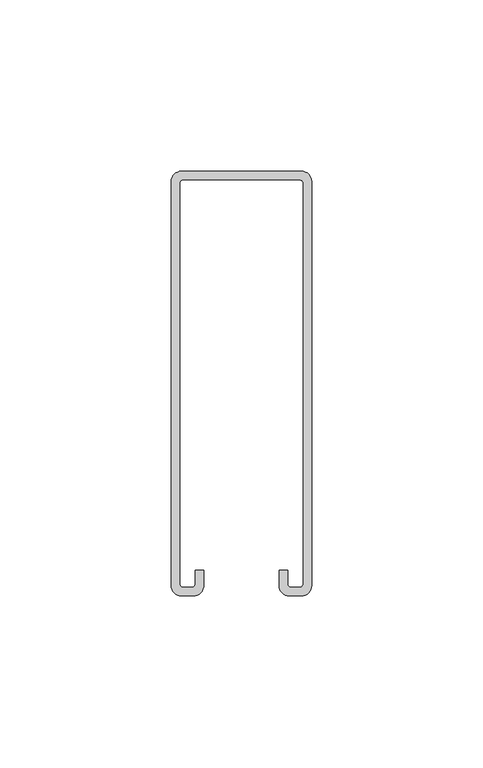
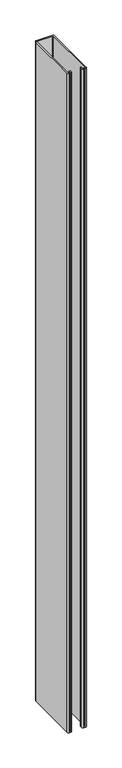
"""IFC4 building model written with IfcOpenShell, lengths in millimetres: proxy geometry, TN_Профиль монтажный : Профиль монтажный 41x124x2,5-6000."""

from ifc_helpers import new_model, si_unit, point, frame_2d, origin, origin_with_axes, place, context, project, spatial, polyline, circle_curve, trimmed, segment, composite_curve, outline, extrude, source, transform, mapped, element, save


def generic_models_93cc7051(model_context):
    return source(origin(), model_context, "Body", "SweptSolid", [
        extrude(outline(composite_curve([segment(trimmed(circle_curve(frame_2d((-17.5, -3.0)), 3.0), [point((-20.5, -3.0))], [point((-17.5, 0.0))], False, "CARTESIAN"), True, "CONTINUOUS"), segment(polyline([(-17.5, 0.0), (17.5, 0.0)]), True, "CONTINUOUS"), segment(trimmed(circle_curve(frame_2d((17.5, -3.0)), 3.0), [point((17.5, 0.0))], [point((20.5, -3.0))], False, "CARTESIAN"), True, "CONTINUOUS"), segment(polyline([(20.5, -3.0), (20.5, -121.0)]), True, "CONTINUOUS"), segment(trimmed(circle_curve(frame_2d((17.5, -121.0)), 3.0), [point((20.5, -121.0))], [point((17.5, -124.0))], False, "CARTESIAN"), True, "CONTINUOUS"), segment(polyline([(17.5, -124.0), (14.0, -124.0)]), True, "CONTINUOUS"), segment(trimmed(circle_curve(frame_2d((14.0, -121.0)), 3.0), [point((14.0, -124.0))], [point((11.0, -121.0))], False, "CARTESIAN"), True, "CONTINUOUS"), segment(polyline([(11.0, -121.0), (11.0, -116.5), (13.5, -116.5), (13.5, -120.5)]), True, "CONTINUOUS"), segment(trimmed(circle_curve(frame_2d((14.5, -120.5)), 1.0), [point((13.5, -120.5))], [point((14.5, -121.5))], True, "CARTESIAN"), True, "CONTINUOUS"), segment(polyline([(14.5, -121.5), (17.0, -121.5)]), True, "CONTINUOUS"), segment(trimmed(circle_curve(frame_2d((17.0, -120.5)), 1.0), [point((17.0, -121.5))], [point((18.0, -120.5))], True, "CARTESIAN"), True, "CONTINUOUS"), segment(polyline([(18.0, -120.5), (18.0, -3.5)]), True, "CONTINUOUS"), segment(trimmed(circle_curve(frame_2d((17.0, -3.5)), 1.0), [point((18.0, -3.5))], [point((17.0, -2.5))], True, "CARTESIAN"), True, "CONTINUOUS"), segment(polyline([(17.0, -2.5), (-17.0, -2.5)]), True, "CONTINUOUS"), segment(trimmed(circle_curve(frame_2d((-17.0, -3.5)), 1.0), [point((-17.0, -2.5))], [point((-18.0, -3.5))], True, "CARTESIAN"), True, "CONTINUOUS"), segment(polyline([(-18.0, -3.5), (-18.0, -120.5)]), True, "CONTINUOUS"), segment(trimmed(circle_curve(frame_2d((-17.0, -120.5)), 1.0), [point((-18.0, -120.5))], [point((-17.0, -121.5))], True, "CARTESIAN"), True, "CONTINUOUS"), segment(polyline([(-17.0, -121.5), (-14.5, -121.5)]), True, "CONTINUOUS"), segment(trimmed(circle_curve(frame_2d((-14.5, -120.5)), 1.0), [point((-14.5, -121.5))], [point((-13.5, -120.5))], True, "CARTESIAN"), True, "CONTINUOUS"), segment(polyline([(-13.5, -120.5), (-13.5, -116.5), (-11.0, -116.5), (-11.0, -120.9588961)]), True, "CONTINUOUS"), segment(trimmed(circle_curve(frame_2d((-14.0411039, -120.9588961)), 3.0411039), [point((-11.0, -120.9588961))], [point((-14.0411039, -124.0))], False, "CARTESIAN"), True, "CONTINUOUS"), segment(polyline([(-14.0411039, -124.0), (-17.5, -124.0)]), True, "CONTINUOUS"), segment(trimmed(circle_curve(frame_2d((-17.5, -121.0)), 3.0), [point((-17.5, -124.0))], [point((-20.5, -121.0))], False, "CARTESIAN"), True, "CONTINUOUS"), segment(polyline([(-20.5, -121.0), (-20.5, -3.0)]), True, "CONTINUOUS")], self_intersect=False)), origin_with_axes(), (0.0, 0.0, 1.0), 1500.0),
    ])


if __name__ == "__main__":
    model = new_model("IFC4")
    model_context = context("Model", 3, world=origin())
    ifc_project = project(units=[si_unit("LENGTHUNIT", "METRE", prefix="MILLI")], contexts=[model_context])
    site = spatial("IfcSite", under=ifc_project)
    building = spatial("IfcBuilding", under=site)
    placement = place(None, origin())
    generic_models_shape = generic_models_93cc7051(model_context)
    element("IfcBuildingElementProxy", 1, Name="TN_Профиль монтажный : Профиль монтажный 41x124x2,5-6000", ObjectType="TN_Профиль монтажный : Профиль монтажный 41x124x2,5-6000", at=placement, inside=building, context=model_context, shape_type="MappedRepresentation", body=[
        mapped(generic_models_shape, transform((0.0, 0.0, 0.0), x_axis=(1.0, 0.0, 0.0), y_axis=(0.0, 1.0, 0.0), z_axis=(0.0, 0.0, 1.0))),
    ])
    save(model, "model.ifc")

# Revit data of these elements
# Type "TN_Профиль монтажный : Профиль монтажный 41x124x2,5-6000"
#   Description = "Профиль монтажный – траверса С-образной формы предназначен для горизонтального и вертикального монтажа тяжелых инженерных систем, оборудования систем вентиляции и кондиционирования, установок электроснабжения, элементов трубопроводов, также для изготовления стенных консолей пристенного монтажа, рам оснований различного типа под оборудование. Возможно замещение на основе сконструированных модулей серийных опор ГОСТ для раскрепления технологических трубопроводов. Рекомендуется для применения в сухих, влажных помещениях и на открытом воздухе."
#   Manufacturer = "ТехноНИКОЛЬ"
#   Model = "Комплектующие к опорам"
#   URL = "https://nav.tn.ru/knowledge-base/polimernye-membrany/opory-pod-oborudovanie-na-ploskoy-krovle/?sphrase_id=266812"
#   ADSK_Обозначение = "ТехноНИКОЛЬ"
#   ADSK_Наименование краткое = "П41x124x2,5"
#   ADSK_Наименование = "Профиль монтажный 41x124x2,5-6000"
#   ADSK_Масса_Текст = ""
#   ADSK_Марка = "П41x124x2,5"
#   ADSK_Код изделия = "690881"
#   ADSK_Завод-изготовитель = "ТехноНИКОЛЬ"
#   ADSK_Единица измерения = "п.м."
#   ADSK_Группирование = "Комплектующие к опорам"
#   ADSK_URL страницы изделия = "https://nav.tn.ru/knowledge-base/polimernye-membrany/opory-pod-oborudovanie-na-ploskoy-krovle/?sphrase_id=266812"
#   ADSK_URL документации изделия = ""
#   Размер_Длина_Вводимая [instance default] = 1000 mm
#   ADSK_Размер_Длина [instance default] = 1000 mm
#   ADSK_Количество [instance default] = 1
#   Тип профиля = 2
#   Профиль монтажный 41х41x2,0 = no
#   Профиль монтажный 41x62x2,5 = no
#   Профиль монтажный 41x124x2,5 = yes
#   ADSK_Материал = TN_СтальГальванизированная_Серый
#   Default Elevation = 0
# Element 1 (IfcBuildingElementProxy, "TN_Профиль монтажный : Профиль монтажный 41x124x2,5-6000")
#   Размер_Длина_Вводимая = 1500 mm
#   ADSK_Размер_Длина = 1500 mm
#   ADSK_Количество = 1.5
#   Materials on its faces: "TN_СтальГальванизированная_Серый"
# Materials
#   "TN_СтальГальванизированная_Серый": class "Типовые", colour RGB 206 210 213, transparency 0, Cost = 0
